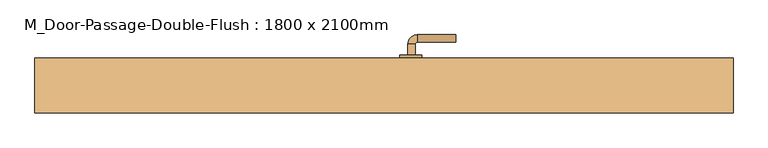
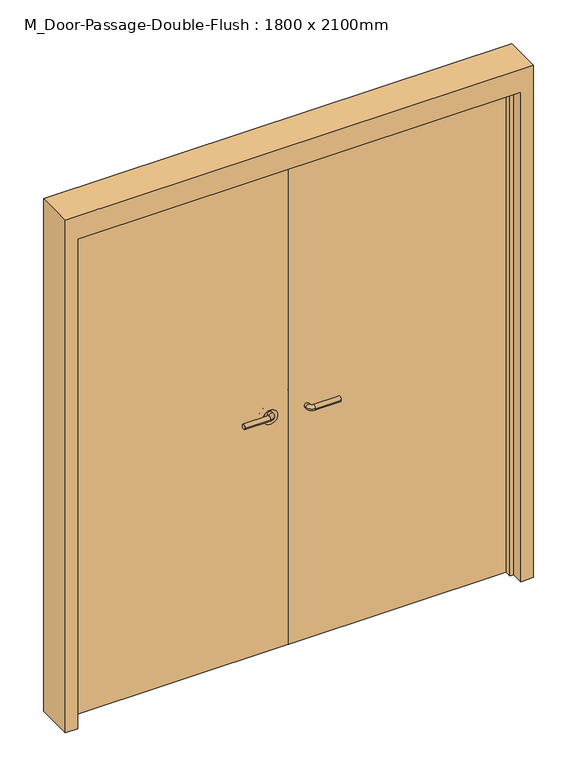
"""IFC4 building model written with IfcOpenShell, lengths in millimetres: door geometry, M_Door-Passage-Double-Flush : 1800 x 2100mm."""

from ifc_helpers import new_model, si_unit, point, frame, frame_2d, origin, origin_with_axes, place, context, project, spatial, polyline, circle_curve, ellipse_curve, trimmed, segment, composite_curve, outline, extrude, faceted_brep, source, transform, mapped, element, save
from ifc_brep_helpers import plane_surface, cylinder_surface, revolved_surface, advanced_brep


def m_door_passage_double_flush_1800_x_2100mm_17443fe2(model_context):
    return source(origin(), model_context, "Body", "SolidModel", [
        advanced_brep(
        [(-65.009375, 102.85, 1016.0), (-85.009375, 102.85, 1016.0), (-65.009375, 72.85, 1016.0), (-85.009375, 72.85, 1016.0), (-90.009375, 67.85, 1016.0), (-90.009375, 47.85, 1016.0), (-195.009375, 47.85, 1016.0), (-195.009375, 67.85, 1016.0)],
        [
            (0, 1, circle_curve(frame((-75.009375, 102.85, 1016.0), z_axis=(0.0, 1.0, 0.0), x_axis=(-1.0, 0.0, 0.0)), 10.0)),
            (1, 0, circle_curve(frame((-75.009375, 102.85, 1016.0), z_axis=(0.0, 1.0, 0.0), x_axis=(-1.0, 0.0, 0.0)), 10.0)),
            (0, 2),
            (2, 3, circle_curve(frame((-75.009375, 72.85, 1016.0), z_axis=(0.0, 1.0, 0.0), x_axis=(-1.0, 0.0, 0.0)), 10.0)),
            (3, 1),
            (3, 2, circle_curve(frame((-75.009375, 72.85, 1016.0), z_axis=(0.0, 1.0, 0.0), x_axis=(-1.0, 0.0, 0.0)), 10.0)),
            (4, 3, circle_curve(frame((-90.009375, 72.85, 1016.0), z_axis=(0.0, 0.0, 1.0), x_axis=(1.0, 0.0, 0.0)), 5.0)),
            (2, 5, circle_curve(frame((-90.009375, 72.85, 1016.0), z_axis=(0.0, 0.0, -1.0), x_axis=(1.0, 0.0, 0.0)), 25.0)),
            (5, 4, circle_curve(frame((-90.009375, 57.85, 1016.0), z_axis=(1.0, 0.0, 0.0), x_axis=(0.0, 1.0, 0.0)), 10.0)),
            (4, 5, circle_curve(frame((-90.009375, 57.85, 1016.0), z_axis=(1.0, 0.0, 0.0), x_axis=(0.0, 1.0, 0.0)), 10.0)),
            (6, 7, circle_curve(frame((-195.009375, 57.85, 1016.0), z_axis=(-1.0, 0.0, 0.0), x_axis=(0.0, 1.0, 0.0)), 10.0)),
            (7, 6, circle_curve(frame((-195.009375, 57.85, 1016.0), z_axis=(-1.0, 0.0, 0.0), x_axis=(0.0, 1.0, 0.0)), 10.0)),
            (5, 6),
            (7, 4),
        ],
        [
            plane_surface(frame((-75.009375, 102.85, 1016.0), z_axis=(0.0, 1.0, 0.0), x_axis=(0.0, 0.0, 1.0))),
            cylinder_surface(frame((-75.009375, 102.85, 1016.0), z_axis=(0.0, 1.0, 0.0), x_axis=(-1.0, 0.0, 0.0)), 10.0),
            revolved_surface(trimmed(ellipse_curve(frame((-75.009375, 72.85, 1016.0), z_axis=(0.0, 1.0, 0.0), x_axis=(-1.0, 0.0, 0.0)), 10.0, 10.0), [point((-65.009375, 72.85, 1016.0))], [point((-85.009375, 72.85, 1016.0))], True, "CARTESIAN"), (-90.009375, 72.85, 1016.0), (0.0, 0.0, -1.0)),
            revolved_surface(trimmed(ellipse_curve(frame((-75.009375, 72.85, 1016.0), z_axis=(0.0, 1.0, 0.0), x_axis=(-1.0, 0.0, 0.0)), 10.0, 10.0), [point((-85.009375, 72.85, 1016.0))], [point((-65.009375, 72.85, 1016.0))], True, "CARTESIAN"), (-90.009375, 72.85, 1016.0), (0.0, 0.0, -1.0)),
            plane_surface(frame((-195.009375, 57.85, 1016.0), z_axis=(-1.0, 0.0, 0.0), x_axis=(0.0, 0.0, 1.0))),
            cylinder_surface(frame((-90.009375, 57.85, 1016.0), z_axis=(1.0, 0.0, 0.0), x_axis=(0.0, 1.0, 0.0)), 10.0),
        ],
        [
            (0, [[1, 2]]),
            (1, [[-1, 3, 4, 5]]),
            (1, [[-2, -5, 6, -3]]),
            (2, [[7, -4, 8, 9]]),
            (3, [[-8, -6, -7, 10]]),
            (4, [[11, 12]]),
            (5, [[-9, 13, -12, 14]]),
            (5, [[-10, -14, -11, -13]]),
        ],
    ),
        extrude(outline(composite_curve([segment(trimmed(circle_curve(frame_2d((1016.0, -72.509375)), 30.0), [point((1016.0, -42.509375))], [point((1016.0, -102.509375))], False, "CARTESIAN"), True, "CONTINUOUS"), segment(trimmed(circle_curve(frame_2d((1016.0, -72.509375)), 30.0), [point((1016.0, -102.509375))], [point((1016.0, -42.509375))], False, "CARTESIAN"), True, "CONTINUOUS")], self_intersect=False)), frame((0.0, 102.85, 0.0), z_axis=(0.0, 1.0, 0.0), x_axis=(0.0, 0.0, 1.0)), (0.0, 0.0, 1.0), 8.0),
        advanced_brep(
        [(-65.009375, 90.95, 1000.0), (-85.009375, 90.95, 1000.0), (-85.009375, 120.95, 1000.0), (-65.009375, 120.95, 1000.0), (-90.009375, 125.95, 1000.0), (-90.009375, 145.95, 1000.0), (-195.009375, 145.95, 1000.0), (-195.009375, 125.95, 1000.0)],
        [
            (0, 1, circle_curve(frame((-75.009375, 90.95, 1000.0), z_axis=(0.0, -1.0, 0.0), x_axis=(-1.0, 0.0, 0.0)), 10.0)),
            (1, 0, circle_curve(frame((-75.009375, 90.95, 1000.0), z_axis=(0.0, -1.0, 0.0), x_axis=(-1.0, 0.0, 0.0)), 10.0)),
            (1, 2),
            (2, 3, circle_curve(frame((-75.009375, 120.95, 1000.0), z_axis=(0.0, -1.0, 0.0), x_axis=(-1.0, 0.0, 0.0)), 10.0)),
            (3, 0),
            (3, 2, circle_curve(frame((-75.009375, 120.95, 1000.0), z_axis=(0.0, -1.0, 0.0), x_axis=(-1.0, 0.0, 0.0)), 10.0)),
            (4, 5, circle_curve(frame((-90.009375, 135.95, 1000.0), z_axis=(1.0, 0.0, 0.0), x_axis=(0.0, -1.0, 0.0)), 10.0)),
            (5, 3, circle_curve(frame((-90.009375, 120.95, 1000.0), z_axis=(0.0, 0.0, -1.0), x_axis=(1.0, 0.0, 0.0)), 25.0)),
            (2, 4, circle_curve(frame((-90.009375, 120.95, 1000.0), z_axis=(0.0, 0.0, 1.0), x_axis=(1.0, 0.0, 0.0)), 5.0)),
            (5, 4, circle_curve(frame((-90.009375, 135.95, 1000.0), z_axis=(1.0, 0.0, 0.0), x_axis=(0.0, -1.0, 0.0)), 10.0)),
            (6, 7, circle_curve(frame((-195.009375, 135.95, 1000.0), z_axis=(-1.0, 0.0, 0.0), x_axis=(0.0, -1.0, 0.0)), 10.0)),
            (7, 6, circle_curve(frame((-195.009375, 135.95, 1000.0), z_axis=(-1.0, 0.0, 0.0), x_axis=(0.0, -1.0, 0.0)), 10.0)),
            (4, 7),
            (6, 5),
        ],
        [
            plane_surface(frame((-75.009375, 90.95, 1000.0), z_axis=(0.0, -1.0, 0.0), x_axis=(0.0, 0.0, 1.0))),
            cylinder_surface(frame((-75.009375, 90.95, 1000.0), z_axis=(0.0, -1.0, 0.0), x_axis=(-1.0, 0.0, 0.0)), 10.0),
            revolved_surface(trimmed(ellipse_curve(frame((-75.009375, 120.95, 1000.0), z_axis=(0.0, 1.0, 0.0), x_axis=(-1.0, 0.0, 0.0)), 10.0, 10.0), [point((-65.009375, 120.95, 1000.0))], [point((-85.009375, 120.95, 1000.0))], True, "CARTESIAN"), (-90.009375, 120.95, 1000.0), (0.0, 0.0, -1.0)),
            revolved_surface(trimmed(ellipse_curve(frame((-75.009375, 120.95, 1000.0), z_axis=(0.0, 1.0, 0.0), x_axis=(-1.0, 0.0, 0.0)), 10.0, 10.0), [point((-85.009375, 120.95, 1000.0))], [point((-65.009375, 120.95, 1000.0))], True, "CARTESIAN"), (-90.009375, 120.95, 1000.0), (0.0, 0.0, -1.0)),
            plane_surface(frame((-195.009375, 135.95, 1000.0), z_axis=(-1.0, 0.0, 0.0), x_axis=(0.0, 0.0, 1.0))),
            cylinder_surface(frame((-90.009375, 135.95, 1000.0), z_axis=(1.0, 0.0, 0.0), x_axis=(0.0, -1.0, 0.0)), 10.0),
        ],
        [
            (0, [[1, 2]]),
            (1, [[3, 4, 5, -2]]),
            (1, [[-5, 6, -3, -1]]),
            (2, [[7, 8, -4, 9]]),
            (3, [[10, -9, -6, -8]]),
            (4, [[11, 12]]),
            (5, [[13, -11, 14, -7]]),
            (5, [[-14, -12, -13, -10]]),
        ],
    ),
        extrude(outline(composite_curve([segment(trimmed(circle_curve(frame_2d((1000.0, -72.509375)), 30.0), [point((1000.0, -42.509375))], [point((1000.0, -102.509375))], False, "CARTESIAN"), True, "CONTINUOUS"), segment(trimmed(circle_curve(frame_2d((1000.0, -72.509375)), 30.0), [point((1000.0, -102.509375))], [point((1000.0, -42.509375))], False, "CARTESIAN"), True, "CONTINUOUS")], self_intersect=False)), frame((0.0, 82.95, 0.0), z_axis=(0.0, 1.0, 0.0), x_axis=(0.0, 0.0, 1.0)), (0.0, 0.0, 1.0), 8.0),
        advanced_brep(
        [(65.009375, 102.85, 1000.0), (85.009375, 102.85, 1000.0), (85.009375, 72.85, 1000.0), (65.009375, 72.85, 1000.0), (90.009375, 67.85, 1000.0), (90.009375, 47.85, 1000.0), (195.009375, 47.85, 1000.0), (195.009375, 67.85, 1000.0)],
        [
            (0, 1, circle_curve(frame((75.009375, 102.85, 1000.0), z_axis=(0.0, 1.0, 0.0), x_axis=(1.0, 0.0, 0.0)), 10.0)),
            (1, 0, circle_curve(frame((75.009375, 102.85, 1000.0), z_axis=(0.0, 1.0, 0.0), x_axis=(1.0, 0.0, 0.0)), 10.0)),
            (1, 2),
            (2, 3, circle_curve(frame((75.009375, 72.85, 1000.0), z_axis=(0.0, 1.0, 0.0), x_axis=(1.0, 0.0, 0.0)), 10.0)),
            (3, 0),
            (3, 2, circle_curve(frame((75.009375, 72.85, 1000.0), z_axis=(0.0, 1.0, 0.0), x_axis=(1.0, 0.0, 0.0)), 10.0)),
            (4, 5, circle_curve(frame((90.009375, 57.85, 1000.0), z_axis=(-1.0, 0.0, 0.0), x_axis=(0.0, 1.0, 0.0)), 10.0)),
            (5, 3, circle_curve(frame((90.009375, 72.85, 1000.0), z_axis=(0.0, 0.0, -1.0), x_axis=(-1.0, 0.0, 0.0)), 25.0)),
            (2, 4, circle_curve(frame((90.009375, 72.85, 1000.0), z_axis=(0.0, 0.0, 1.0), x_axis=(-1.0, 0.0, 0.0)), 5.0)),
            (5, 4, circle_curve(frame((90.009375, 57.85, 1000.0), z_axis=(-1.0, 0.0, 0.0), x_axis=(0.0, 1.0, 0.0)), 10.0)),
            (6, 7, circle_curve(frame((195.009375, 57.85, 1000.0), z_axis=(1.0, 0.0, 0.0), x_axis=(0.0, 1.0, 0.0)), 10.0)),
            (7, 6, circle_curve(frame((195.009375, 57.85, 1000.0), z_axis=(1.0, 0.0, 0.0), x_axis=(0.0, 1.0, 0.0)), 10.0)),
            (4, 7),
            (6, 5),
        ],
        [
            plane_surface(frame((75.009375, 102.85, 1000.0), z_axis=(0.0, 1.0, 0.0), x_axis=(0.0, 0.0, 1.0))),
            cylinder_surface(frame((75.009375, 102.85, 1000.0), z_axis=(0.0, 1.0, 0.0), x_axis=(1.0, 0.0, 0.0)), 10.0),
            revolved_surface(trimmed(ellipse_curve(frame((75.009375, 72.85, 1000.0), z_axis=(0.0, -1.0, 0.0), x_axis=(1.0, 0.0, 0.0)), 10.0, 10.0), [point((65.009375, 72.85, 1000.0))], [point((85.009375, 72.85, 1000.0))], True, "CARTESIAN"), (90.009375, 72.85, 1000.0), (0.0, 0.0, -1.0)),
            revolved_surface(trimmed(ellipse_curve(frame((75.009375, 72.85, 1000.0), z_axis=(0.0, -1.0, 0.0), x_axis=(1.0, 0.0, 0.0)), 10.0, 10.0), [point((85.009375, 72.85, 1000.0))], [point((65.009375, 72.85, 1000.0))], True, "CARTESIAN"), (90.009375, 72.85, 1000.0), (0.0, 0.0, -1.0)),
            plane_surface(frame((195.009375, 57.85, 1000.0), z_axis=(1.0, 0.0, 0.0), x_axis=(0.0, 0.0, 1.0))),
            cylinder_surface(frame((90.009375, 57.85, 1000.0), z_axis=(-1.0, 0.0, 0.0), x_axis=(0.0, 1.0, 0.0)), 10.0),
        ],
        [
            (0, [[1, 2]]),
            (1, [[3, 4, 5, -2]]),
            (1, [[-5, 6, -3, -1]]),
            (2, [[7, 8, -4, 9]]),
            (3, [[10, -9, -6, -8]]),
            (4, [[11, 12]]),
            (5, [[13, -11, 14, -7]]),
            (5, [[-14, -12, -13, -10]]),
        ],
    ),
        extrude(outline(composite_curve([segment(trimmed(circle_curve(frame_2d((1000.0, 72.509375)), 30.0), [point((1000.0, 42.509375))], [point((1000.0, 102.509375))], False, "CARTESIAN"), True, "CONTINUOUS"), segment(trimmed(circle_curve(frame_2d((1000.0, 72.509375)), 30.0), [point((1000.0, 102.509375))], [point((1000.0, 42.509375))], False, "CARTESIAN"), True, "CONTINUOUS")], self_intersect=False)), frame((0.0, 102.85, 0.0), z_axis=(0.0, 1.0, 0.0), x_axis=(0.0, 0.0, 1.0)), (0.0, 0.0, 1.0), 8.0),
        advanced_brep(
        [(65.009375, 163.85, 1000.0), (85.009375, 163.85, 1000.0), (65.009375, 193.85, 1000.0), (85.009375, 193.85, 1000.0), (90.009375, 198.85, 1000.0), (90.009375, 218.85, 1000.0), (195.009375, 218.85, 1000.0), (195.009375, 198.85, 1000.0)],
        [
            (0, 1, circle_curve(frame((75.009375, 163.85, 1000.0), z_axis=(0.0, -1.0, 0.0), x_axis=(1.0, 0.0, 0.0)), 10.0)),
            (1, 0, circle_curve(frame((75.009375, 163.85, 1000.0), z_axis=(0.0, -1.0, 0.0), x_axis=(1.0, 0.0, 0.0)), 10.0)),
            (0, 2),
            (2, 3, circle_curve(frame((75.009375, 193.85, 1000.0), z_axis=(0.0, -1.0, 0.0), x_axis=(1.0, 0.0, 0.0)), 10.0)),
            (3, 1),
            (3, 2, circle_curve(frame((75.009375, 193.85, 1000.0), z_axis=(0.0, -1.0, 0.0), x_axis=(1.0, 0.0, 0.0)), 10.0)),
            (4, 3, circle_curve(frame((90.009375, 193.85, 1000.0), z_axis=(0.0, 0.0, 1.0), x_axis=(-1.0, 0.0, 0.0)), 5.0)),
            (2, 5, circle_curve(frame((90.009375, 193.85, 1000.0), z_axis=(0.0, 0.0, -1.0), x_axis=(-1.0, 0.0, 0.0)), 25.0)),
            (5, 4, circle_curve(frame((90.009375, 208.85, 1000.0), z_axis=(-1.0, 0.0, 0.0), x_axis=(0.0, -1.0, 0.0)), 10.0)),
            (4, 5, circle_curve(frame((90.009375, 208.85, 1000.0), z_axis=(-1.0, 0.0, 0.0), x_axis=(0.0, -1.0, 0.0)), 10.0)),
            (6, 7, circle_curve(frame((195.009375, 208.85, 1000.0), z_axis=(1.0, 0.0, 0.0), x_axis=(0.0, -1.0, 0.0)), 10.0)),
            (7, 6, circle_curve(frame((195.009375, 208.85, 1000.0), z_axis=(1.0, 0.0, 0.0), x_axis=(0.0, -1.0, 0.0)), 10.0)),
            (5, 6),
            (7, 4),
        ],
        [
            plane_surface(frame((75.009375, 163.85, 1000.0), z_axis=(0.0, -1.0, 0.0), x_axis=(0.0, 0.0, 1.0))),
            cylinder_surface(frame((75.009375, 163.85, 1000.0), z_axis=(0.0, -1.0, 0.0), x_axis=(1.0, 0.0, 0.0)), 10.0),
            revolved_surface(trimmed(ellipse_curve(frame((75.009375, 193.85, 1000.0), z_axis=(0.0, -1.0, 0.0), x_axis=(1.0, 0.0, 0.0)), 10.0, 10.0), [point((65.009375, 193.85, 1000.0))], [point((85.009375, 193.85, 1000.0))], True, "CARTESIAN"), (90.009375, 193.85, 1000.0), (0.0, 0.0, -1.0)),
            revolved_surface(trimmed(ellipse_curve(frame((75.009375, 193.85, 1000.0), z_axis=(0.0, -1.0, 0.0), x_axis=(1.0, 0.0, 0.0)), 10.0, 10.0), [point((85.009375, 193.85, 1000.0))], [point((65.009375, 193.85, 1000.0))], True, "CARTESIAN"), (90.009375, 193.85, 1000.0), (0.0, 0.0, -1.0)),
            plane_surface(frame((195.009375, 208.85, 1000.0), z_axis=(1.0, 0.0, 0.0), x_axis=(0.0, 0.0, 1.0))),
            cylinder_surface(frame((90.009375, 208.85, 1000.0), z_axis=(-1.0, 0.0, 0.0), x_axis=(0.0, -1.0, 0.0)), 10.0),
        ],
        [
            (0, [[1, 2]]),
            (1, [[-1, 3, 4, 5]]),
            (1, [[-2, -5, 6, -3]]),
            (2, [[7, -4, 8, 9]]),
            (3, [[-8, -6, -7, 10]]),
            (4, [[11, 12]]),
            (5, [[-9, 13, -12, 14]]),
            (5, [[-10, -14, -11, -13]]),
        ],
    ),
        extrude(outline(composite_curve([segment(trimmed(circle_curve(frame_2d((1000.0, 72.509375)), 30.0), [point((1000.0, 42.509375))], [point((1000.0, 102.509375))], False, "CARTESIAN"), True, "CONTINUOUS"), segment(trimmed(circle_curve(frame_2d((1000.0, 72.509375)), 30.0), [point((1000.0, 102.509375))], [point((1000.0, 42.509375))], False, "CARTESIAN"), True, "CONTINUOUS")], self_intersect=False)), frame((0.0, 155.85, 0.0), z_axis=(0.0, 1.0, 0.0), x_axis=(0.0, 0.0, 1.0)), (0.0, 0.0, 1.0), 8.0),
        extrude(outline(polyline([(900.0, 82.95), (1.5875, 82.95), (1.5875, 110.85), (900.0, 110.85), (900.0, 82.95)])), origin_with_axes(), (0.0, 0.0, 1.0), 2100.0),
        extrude(outline(polyline([(-1.5875, 82.95), (-900.0, 82.95), (-900.0, 110.85), (-1.5875, 110.85), (-1.5875, 82.95)])), origin_with_axes(), (0.0, 0.0, 1.0), 2100.0),
        faceted_brep([(900.0, 106.0875, 0.0), (900.0, 155.85, 0.0), (950.0, 155.85, 0.0), (950.0, 5.85, 0.0), (900.0, 5.85, 0.0), (900.0, 55.0625, 0.0), (884.125, 55.0625, 0.0), (884.125, 106.0875, 0.0), (900.0, 106.0875, 2100.0), (900.0, 155.85, 2100.0), (-900.0, 155.85, 2100.0), (-900.0, 155.85, 0.0), (-950.0, 155.85, 0.0), (-950.0, 155.85, 2200.0), (950.0, 155.85, 2200.0), (950.0, 5.85, 2200.0), (-950.0, 5.85, 2200.0), (-950.0, 5.85, 0.0), (-900.0, 5.85, 0.0), (-900.0, 5.85, 2100.0), (900.0, 5.85, 2100.0), (900.0, 55.0625, 2100.0), (-900.0, 55.0625, 2100.0), (-900.0, 55.0625, 0.0), (-884.125, 55.0625, 0.0), (-884.125, 55.0625, 2084.125), (884.125, 55.0625, 2084.125), (884.125, 106.0875, 2084.125), (-884.125, 106.0875, 2084.125), (-884.125, 106.0875, 0.0), (-900.0, 106.0875, 0.0), (-900.0, 106.0875, 2100.0)], [[[0, 1, 2, 3, 4, 5, 6, 7]], [[1, 0, 8, 9]], [[2, 1, 9, 10, 11, 12, 13, 14]], [[3, 2, 14, 15]], [[4, 3, 15, 16, 17, 18, 19, 20]], [[5, 4, 20, 21]], [[6, 5, 21, 22, 23, 24, 25, 26]], [[7, 6, 26, 27]], [[0, 7, 27, 28, 29, 30, 31, 8]], [[9, 8, 31, 10]], [[20, 19, 22, 21]], [[26, 25, 28, 27]], [[12, 11, 30, 29, 24, 23, 18, 17]], [[11, 10, 31, 30]], [[13, 12, 17, 16]], [[19, 18, 23, 22]], [[25, 24, 29, 28]], [[15, 14, 13, 16]]]),
    ])


if __name__ == "__main__":
    model = new_model("IFC4")
    model_context = context("Model", 3, world=origin())
    ifc_project = project(units=[si_unit("LENGTHUNIT", "METRE", prefix="MILLI")], contexts=[model_context])
    site = spatial("IfcSite", under=ifc_project)
    building = spatial("IfcBuilding", under=site)
    placement = place(None, origin())
    m_door_passage_double_flush_1800_x_2100mm_shape = m_door_passage_double_flush_1800_x_2100mm_17443fe2(model_context)
    element("IfcDoor", 1, ObjectType="M_Door-Passage-Double-Flush : 1800 x 2100mm", at=placement, inside=building, context=model_context, shape_type="MappedRepresentation", body=[
        mapped(m_door_passage_double_flush_1800_x_2100mm_shape, transform((0.0, 0.0, 0.0), x_axis=(1.0, 0.0, 0.0), y_axis=(0.0, 1.0, 0.0), z_axis=(0.0, 0.0, 1.0))),
    ])
    save(model, "model.ifc")

# Revit data of these elements
# Type "M_Door-Passage-Double-Flush : 1800 x 2100mm"
#   Type Mark = "34"
#   Assembly Code = "B2030200"
#   Analytic Construction = "Metal"
#   Thickness = 45 mm
#   Thermal Resistance (R) = 0.270118 (m²·K)/W
#   Swing Angle [instance default] = 90.00°
#   Strike Height = 1000 mm
#   SinglePanelWidth = 900 mm
#   Rough Width [instance default] = 1900 mm
#   Rough Height [instance default] = 2200 mm
#   MFOpeningHeight [instance default] = 100 mm
#   MFOpeningWidth [instance default] = 100 mm
#   Inset Calculate [instance default] = 105 mm
#   Masonry Inset [instance default] = 25 mm
#   Height = 2100 mm
#   Width = 1800 mm
#   Heat Transfer Coefficient (U) = 3.70223 W/(m²·K)
#   Masonry Frame Depth = 150 mm
#   Masonry Frame [instance default] = yes
#   Function = 1
#   Dry Wall Frame [instance default] = no
#   Panel Material = Metal Door - Brindle
#   Frame Material = Metal - Painted - Grey
#   Door Handle Material = Aluminum
#   Visual Light Transmittance = 0
#   Solar Heat Gain Coefficient = 0
#   Wall Closure = (empty or 0)
# Element 1 (IfcDoor, "M_Door-Passage-Double-Flush : 1800 x 2100mm")
#   Materials on its faces: "Aluminum", "Metal - Painted - Grey", "Metal Door - Brindle"
# Materials
#   "Metal Door - Brindle": class "Paint", colour RGB 164 133 98, transparency 0
#   "Metal - Painted - Grey": class "Paint", colour RGB 104 104 104, transparency 0
#   "Aluminum": class "Metal", colour RGB 244 245 246, transparency 0, Description = "Aluminum 6061", Cost = 0
